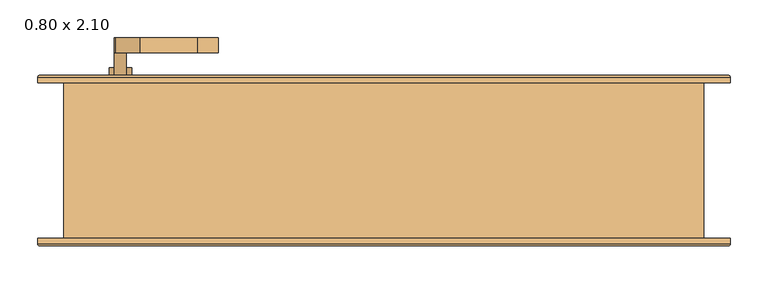
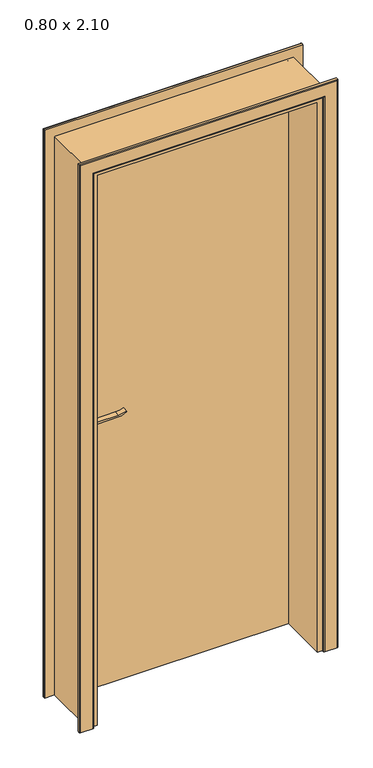
"""IFC4 building model written with IfcOpenShell, lengths in millimetres: door geometry, .CC_ND 300_PORTA SIMPLES DE ABRIR_COM EXTENSÃO : 0.80 x 2.10."""

from ifc_helpers import new_model, si_unit, point, frame, frame_2d, origin, origin_with_axes, place, context, project, spatial, polyline, circle_curve, ellipse_curve, trimmed, segment, composite_curve, outline, extrude, faceted_brep, source, transform, mapped, element, save
from ifc_brep_helpers import plane_surface, cylinder_surface, advanced_brep


def door_0_80_x_2_10_4cab1925(model_context):
    return source(origin(), model_context, "Body", "SolidModel", [
        extrude(outline(composite_curve([segment(trimmed(circle_curve(frame_2d((964.5, -350.0)), 15.0), [point((964.5, -335.0))], [point((964.5, -365.0))], False, "CARTESIAN"), True, "CONTINUOUS"), segment(trimmed(circle_curve(frame_2d((964.5, -350.0)), 15.0), [point((964.5, -365.0))], [point((964.5, -335.0))], False, "CARTESIAN"), True, "CONTINUOUS")], self_intersect=False)), frame((0.0, 110.7, 0.0), z_axis=(0.0, 1.0, 0.0), x_axis=(0.0, 0.0, 1.0)), (0.0, 0.0, 1.0), 10.0),
        extrude(outline(composite_curve([segment(trimmed(circle_curve(frame_2d((964.5, -350.0)), 15.0), [point((964.5, -335.0))], [point((964.5, -365.0))], False, "CARTESIAN"), True, "CONTINUOUS"), segment(trimmed(circle_curve(frame_2d((964.5, -350.0)), 15.0), [point((964.5, -365.0))], [point((964.5, -335.0))], False, "CARTESIAN"), True, "CONTINUOUS")], self_intersect=False)), frame((0.0, 50.7, 0.0), z_axis=(0.0, 1.0, 0.0), x_axis=(0.0, 0.0, 1.0)), (0.0, 0.0, 1.0), 10.0),
        extrude(outline(composite_curve([segment(trimmed(circle_curve(frame_2d((1024.5, -350.0)), 8.0), [point((1029.1523287, -356.5081363))], [point((1024.5, -342.0))], False, "CARTESIAN"), True, "CONTINUOUS"), segment(trimmed(circle_curve(frame_2d((1019.3738613, -324.6138099)), 18.1261387), [point((1024.5, -342.0))], [point((1037.5, -324.6138099))], True, "CARTESIAN"), True, "CONTINUOUS"), segment(polyline([(1037.5, -324.6138099), (1037.5, -248.3564091)]), True, "CONTINUOUS"), segment(trimmed(circle_curve(frame_2d((1096.7709207, -251.9396612)), 59.3791355), [point((1037.5, -248.3564091))], [point((1046.7135558, -220.0))], False, "CARTESIAN"), True, "CONTINUOUS"), segment(polyline([(1046.7135558, -220.0), (1049.5, -220.0)]), True, "CONTINUOUS"), segment(trimmed(circle_curve(frame_2d((1127.7850638, -248.4227909)), 83.2850902), [point((1049.5, -220.0))], [point((1044.5, -248.3564091))], True, "CARTESIAN"), True, "CONTINUOUS"), segment(polyline([(1044.5, -248.3564091), (1044.5, -324.6325667)]), True, "CONTINUOUS"), segment(trimmed(circle_curve(frame_2d((1007.2555521, -326.3324871)), 37.2832219), [point((1044.5, -324.6325667))], [point((1029.1523287, -356.5081363))], False, "CARTESIAN"), True, "CONTINUOUS")], self_intersect=False)), frame((0.0, 140.7, 0.0), z_axis=(0.0, 1.0, 0.0), x_axis=(0.0, 0.0, 1.0)), (0.0, 0.0, 1.0), 20.0),
        extrude(outline(composite_curve([segment(trimmed(circle_curve(frame_2d((1019.3738682, -324.6138122)), 18.1261318), [point((1024.4999903, -342.0))], [point((1037.5, -324.6138122))], True, "CARTESIAN"), True, "CONTINUOUS"), segment(polyline([(1037.5, -324.6138122), (1037.5, -248.3564091)]), True, "CONTINUOUS"), segment(trimmed(circle_curve(frame_2d((1096.7709207, -251.9396612)), 59.3791355), [point((1037.5, -248.3564091))], [point((1046.7135558, -220.0))], False, "CARTESIAN"), True, "CONTINUOUS"), segment(polyline([(1046.7135558, -220.0), (1049.5, -220.0)]), True, "CONTINUOUS"), segment(trimmed(circle_curve(frame_2d((1127.7850638, -248.4227909)), 83.2850902), [point((1049.5, -220.0))], [point((1044.5, -248.3564091))], True, "CARTESIAN"), True, "CONTINUOUS"), segment(polyline([(1044.5, -248.3564091), (1044.5, -324.6325667)]), True, "CONTINUOUS"), segment(trimmed(circle_curve(frame_2d((1007.2555521, -326.3324871)), 37.2832219), [point((1044.5, -324.6325667))], [point((1029.1523287, -356.5081363))], False, "CARTESIAN"), True, "CONTINUOUS"), segment(trimmed(circle_curve(frame_2d((1024.5, -350.0)), 8.0), [point((1029.1523287, -356.5081363))], [point((1024.4999903, -342.0))], False, "CARTESIAN"), True, "CONTINUOUS")], self_intersect=False)), frame((0.0, 10.7, 0.0), z_axis=(0.0, 1.0, 0.0), x_axis=(0.0, 0.0, 1.0)), (0.0, 0.0, 1.0), 20.0),
        extrude(outline(composite_curve([segment(trimmed(circle_curve(frame_2d((1024.5, -350.0)), 8.0), [point((1024.5, -342.0))], [point((1024.5, -358.0))], False, "CARTESIAN"), True, "CONTINUOUS"), segment(trimmed(circle_curve(frame_2d((1024.5, -350.0)), 8.0), [point((1024.5, -358.0))], [point((1024.5, -342.0))], False, "CARTESIAN"), True, "CONTINUOUS")], self_intersect=False)), frame((0.0, 110.7, 0.0), z_axis=(0.0, 1.0, 0.0), x_axis=(0.0, 0.0, 1.0)), (0.0, 0.0, 1.0), 30.0),
        extrude(outline(composite_curve([segment(trimmed(circle_curve(frame_2d((1024.5, -350.0)), 8.0), [point((1024.5, -342.0))], [point((1024.5, -358.0))], False, "CARTESIAN"), True, "CONTINUOUS"), segment(trimmed(circle_curve(frame_2d((1024.5, -350.0)), 8.0), [point((1024.5, -358.0))], [point((1024.5, -342.0))], False, "CARTESIAN"), True, "CONTINUOUS")], self_intersect=False)), frame((0.0, 30.7, 0.0), z_axis=(0.0, 1.0, 0.0), x_axis=(0.0, 0.0, 1.0)), (0.0, 0.0, 1.0), 30.0),
        extrude(outline(composite_curve([segment(trimmed(circle_curve(frame_2d((954.5, -350.0)), 25.0), [point((954.5, -375.0))], [point((954.5, -325.0))], False, "CARTESIAN"), True, "CONTINUOUS"), segment(polyline([(954.5, -325.0), (1024.5, -325.0)]), True, "CONTINUOUS"), segment(trimmed(circle_curve(frame_2d((1024.5, -350.0)), 25.0), [point((1024.5, -325.0))], [point((1024.5, -375.0))], False, "CARTESIAN"), True, "CONTINUOUS"), segment(polyline([(1024.5, -375.0), (954.5, -375.0)]), True, "CONTINUOUS")], self_intersect=False)), frame((0.0, 100.7, 0.0), z_axis=(0.0, 1.0, 0.0), x_axis=(0.0, 0.0, 1.0)), (0.0, 0.0, 1.0), 10.0),
        extrude(outline(composite_curve([segment(trimmed(circle_curve(frame_2d((954.5, -350.0)), 25.0), [point((954.5, -375.0))], [point((954.5, -325.0))], False, "CARTESIAN"), True, "CONTINUOUS"), segment(polyline([(954.5, -325.0), (1024.5, -325.0)]), True, "CONTINUOUS"), segment(trimmed(circle_curve(frame_2d((1024.5, -350.0)), 25.0), [point((1024.5, -325.0))], [point((1024.5, -375.0))], False, "CARTESIAN"), True, "CONTINUOUS"), segment(polyline([(1024.5, -375.0), (954.5, -375.0)]), True, "CONTINUOUS")], self_intersect=False)), frame((0.0, 60.7, 0.0), z_axis=(0.0, 1.0, 0.0), x_axis=(0.0, 0.0, 1.0)), (0.0, 0.0, 1.0), 10.0),
        advanced_brep(
        [(-460.0, 100.7, 0.0), (-460.0, 107.7, 0.0), (-457.0, 110.7, 0.0), (-413.0, 110.7, 0.0), (-410.0, 107.7, 0.0), (-410.0, 100.7, 0.0), (-410.0, 100.7, 2085.0), (410.0, 100.7, 2085.0), (410.0, 100.7, 0.0), (460.0, 100.7, 0.0), (460.0, 100.7, 2135.0), (-460.0, 100.7, 2135.0), (-410.0, 107.7, 2085.0), (-413.0, 110.7, 2088.0), (-457.0, 110.7, 2132.0), (457.0, 110.7, 2132.0), (457.0, 110.7, 0.0), (413.0, 110.7, 0.0), (413.0, 110.7, 2088.0), (-460.0, 107.7, 2135.0), (460.0, 107.7, 0.0), (460.0, 107.7, 2135.0), (410.0, 107.7, 0.0), (410.0, 107.7, 2085.0)],
        [
            (0, 1),
            (1, 2, circle_curve(frame((-457.0, 107.7, 0.0), z_axis=(0.0, 0.0, -1.0), x_axis=(1.0, 0.0, 0.0)), 3.0)),
            (2, 3),
            (3, 4, circle_curve(frame((-413.0, 107.7, 0.0), z_axis=(0.0, 0.0, -1.0), x_axis=(1.0, 0.0, 0.0)), 3.0)),
            (4, 5),
            (5, 0),
            (5, 6),
            (6, 7),
            (7, 8),
            (8, 9),
            (9, 10),
            (10, 11),
            (11, 0),
            (4, 12),
            (12, 6),
            (3, 13),
            (13, 12, ellipse_curve(frame((-413.0, 107.7, 2088.0), z_axis=(-0.7071067811865475, 0.0, -0.7071067811865475), x_axis=(0.7071067811865474, 0.0, -0.7071067811865476)), 4.2426407, 3.0)),
            (2, 14),
            (14, 15),
            (15, 16),
            (16, 17),
            (17, 18),
            (18, 13),
            (1, 19),
            (19, 14, ellipse_curve(frame((-457.0, 107.7, 2132.0), z_axis=(-0.7071067811865475, 0.0, -0.7071067811865475), x_axis=(0.7071067811865474, 0.0, -0.7071067811865476)), 4.2426407, 3.0)),
            (11, 19),
            (9, 20),
            (20, 21),
            (21, 10),
            (8, 22),
            (22, 17, circle_curve(frame((413.0, 107.7, 0.0), z_axis=(0.0, 0.0, -1.0), x_axis=(-1.0, 0.0, 0.0)), 3.0)),
            (16, 20, circle_curve(frame((457.0, 107.7, 0.0), z_axis=(0.0, 0.0, -1.0), x_axis=(-1.0, 0.0, 0.0)), 3.0)),
            (23, 22),
            (7, 23),
            (23, 18, ellipse_curve(frame((413.0, 107.7, 2088.0), z_axis=(0.7071067811865475, 0.0, -0.7071067811865475), x_axis=(0.7071067811865474, 0.0, 0.7071067811865476)), 4.2426407, 3.0)),
            (15, 21, ellipse_curve(frame((457.0, 107.7, 2132.0), z_axis=(0.7071067811865475, 0.0, -0.7071067811865475), x_axis=(0.7071067811865474, 0.0, 0.7071067811865476)), 4.2426407, 3.0)),
            (12, 23),
            (21, 19),
        ],
        [
            plane_surface(frame((-410.0, 100.7, 0.0), z_axis=(0.0, 0.0, -1.0), x_axis=(0.0, -1.0, 0.0))),
            plane_surface(frame((-460.0, 100.7, 0.0), z_axis=(0.0, -1.0, 0.0), x_axis=(0.0, 0.0, 1.0))),
            plane_surface(frame((-410.0, 100.7, 0.0), z_axis=(1.0, 0.0, 0.0), x_axis=(0.0, 0.0, 1.0))),
            cylinder_surface(frame((-413.0, 107.7, 0.0), z_axis=(0.0, 0.0, -1.0), x_axis=(1.0, 0.0, 0.0)), 3.0),
            plane_surface(frame((-413.0, 110.7, 0.0), z_axis=(0.0, 1.0, 0.0), x_axis=(0.0, 0.0, 1.0))),
            cylinder_surface(frame((-457.0, 107.7, 0.0), z_axis=(0.0, 0.0, -1.0), x_axis=(1.0, 0.0, 0.0)), 3.0),
            plane_surface(frame((-460.0, 107.7, 0.0), z_axis=(-1.0, 0.0, 0.0), x_axis=(0.0, 0.0, 1.0))),
            plane_surface(frame((460.0, 107.7, 2135.0), z_axis=(1.0, 0.0, 0.0), x_axis=(0.0, 0.0, -1.0))),
            plane_surface(frame((410.0, 100.7, 0.0), z_axis=(0.0, 0.0, -1.0), x_axis=(0.0, -1.0, 0.0))),
            plane_surface(frame((410.0, 100.7, 2085.0), z_axis=(-1.0, 0.0, 0.0), x_axis=(0.0, 0.0, -1.0))),
            cylinder_surface(frame((413.0, 107.7, 2085.0), z_axis=(0.0, 0.0, 1.0), x_axis=(-1.0, 0.0, 0.0)), 3.0),
            cylinder_surface(frame((457.0, 107.7, 2085.0), z_axis=(0.0, 0.0, 1.0), x_axis=(-1.0, 0.0, 0.0)), 3.0),
            plane_surface(frame((-410.0, 100.7, 2085.0), z_axis=(0.0, 0.0, -1.0), x_axis=(1.0, 0.0, 0.0))),
            plane_surface(frame((-460.0, 107.7, 2135.0), z_axis=(0.0, 0.0, 1.0), x_axis=(1.0, 0.0, 0.0))),
            cylinder_surface(frame((-410.0, 107.7, 2088.0), z_axis=(-1.0, 0.0, 0.0), x_axis=(0.0, 0.0, -1.0)), 3.0),
            cylinder_surface(frame((-410.0, 107.7, 2132.0), z_axis=(-1.0, 0.0, 0.0), x_axis=(0.0, 0.0, -1.0)), 3.0),
        ],
        [
            (0, [[1, 2, 3, 4, 5, 6]]),
            (1, [[7, 8, 9, 10, 11, 12, 13, -6]]),
            (2, [[14, 15, -7, -5]]),
            (3, [[16, 17, -14, -4]]),
            (4, [[18, 19, 20, 21, 22, 23, -16, -3]]),
            (5, [[24, 25, -18, -2]]),
            (6, [[-13, 26, -24, -1]]),
            (7, [[-11, 27, 28, 29]]),
            (8, [[-10, 30, 31, -21, 32, -27]]),
            (9, [[33, -30, -9, 34]]),
            (10, [[-22, -31, -33, 35]]),
            (11, [[-28, -32, -20, 36]]),
            (12, [[37, -34, -8, -15]]),
            (13, [[-12, -29, 38, -26]]),
            (14, [[-23, -35, -37, -17]]),
            (15, [[-38, -36, -19, -25]]),
        ],
    ),
        advanced_brep(
        [(460.0, -106.0, 0.0), (460.0, -113.0342217, 0.0), (457.0342217, -116.0, 0.0), (412.9842717, -116.0, 0.0), (410.0, -113.0157283, 0.0), (410.0, -106.0, 0.0), (410.0, -106.0, 2085.0), (-410.0, -106.0, 2085.0), (-410.0, -106.0, 0.0), (-460.0, -106.0, 0.0), (-460.0, -106.0, 2135.0), (460.0, -106.0, 2135.0), (410.0, -113.0157283, 2085.0), (412.9842717, -116.0, 2087.9842717), (457.0342217, -116.0, 2132.0342217), (-457.0342217, -116.0, 2132.0342217), (-457.0342217, -116.0, 0.0), (-412.9842717, -116.0, 0.0), (-412.9842717, -116.0, 2087.9842717), (460.0, -113.0342217, 2135.0), (-460.0, -113.0342217, 0.0), (-460.0, -113.0342217, 2135.0), (-410.0, -113.0157283, 0.0), (-410.0, -113.0157283, 2085.0)],
        [
            (0, 1),
            (1, 2, circle_curve(frame((457.0342217, -113.0342217, 0.0), z_axis=(0.0, 0.0, -1.0), x_axis=(1.0, 0.0, 0.0)), 2.9657783)),
            (2, 3),
            (3, 4, circle_curve(frame((412.9842717, -113.0157283, 0.0), z_axis=(0.0, 0.0, -1.0), x_axis=(1.0, 0.0, 0.0)), 2.9842717)),
            (4, 5),
            (5, 0),
            (5, 6),
            (6, 7),
            (7, 8),
            (8, 9),
            (9, 10),
            (10, 11),
            (11, 0),
            (4, 12),
            (12, 6),
            (3, 13),
            (13, 12, ellipse_curve(frame((412.9842717, -113.0157283, 2087.9842717), z_axis=(0.7071067811865475, 0.0, -0.7071067811865475), x_axis=(-0.7071067811865474, 0.0, -0.7071067811865476)), 4.2203975, 2.9842717)),
            (2, 14),
            (14, 15),
            (15, 16),
            (16, 17),
            (17, 18),
            (18, 13),
            (1, 19),
            (19, 14, ellipse_curve(frame((457.0342217, -113.0342217, 2132.0342217), z_axis=(0.7071067811865475, 0.0, -0.7071067811865475), x_axis=(-0.7071067811865474, 0.0, -0.7071067811865476)), 4.1942438, 2.9657783)),
            (11, 19),
            (9, 20),
            (20, 21),
            (21, 10),
            (8, 22),
            (22, 17, circle_curve(frame((-412.9842717, -113.0157283, 0.0), z_axis=(0.0, 0.0, -1.0), x_axis=(-1.0, 0.0, 0.0)), 2.9842717)),
            (16, 20, circle_curve(frame((-457.0342217, -113.0342217, 0.0), z_axis=(0.0, 0.0, -1.0), x_axis=(-1.0, 0.0, 0.0)), 2.9657783)),
            (23, 22),
            (7, 23),
            (23, 18, ellipse_curve(frame((-412.9842717, -113.0157283, 2087.9842717), z_axis=(-0.7071067811865475, 0.0, -0.7071067811865475), x_axis=(-0.7071067811865474, 0.0, 0.7071067811865476)), 4.2203975, 2.9842717)),
            (15, 21, ellipse_curve(frame((-457.0342217, -113.0342217, 2132.0342217), z_axis=(-0.7071067811865475, 0.0, -0.7071067811865475), x_axis=(-0.7071067811865474, 0.0, 0.7071067811865476)), 4.1942438, 2.9657783)),
            (12, 23),
            (21, 19),
        ],
        [
            plane_surface(frame((410.0, -106.0, 0.0), z_axis=(0.0, 0.0, -1.0), x_axis=(0.0, -1.0, 0.0))),
            plane_surface(frame((460.0, -106.0, 0.0), z_axis=(0.0, 1.0, 0.0), x_axis=(0.0, 0.0, 1.0))),
            plane_surface(frame((410.0, -106.0, 0.0), z_axis=(-1.0, 0.0, 0.0), x_axis=(0.0, 0.0, 1.0))),
            cylinder_surface(frame((412.9842717, -113.0157283, 0.0), z_axis=(0.0, 0.0, -1.0), x_axis=(1.0, 0.0, 0.0)), 2.9842717),
            plane_surface(frame((412.9842717, -116.0, 0.0), z_axis=(0.0, -1.0, 0.0), x_axis=(0.0, 0.0, 1.0))),
            cylinder_surface(frame((457.0342217, -113.0342217, 0.0), z_axis=(0.0, 0.0, -1.0), x_axis=(1.0, 0.0, 0.0)), 2.9657783),
            plane_surface(frame((460.0, -113.0342217, 0.0), z_axis=(1.0, 0.0, 0.0), x_axis=(0.0, 0.0, 1.0))),
            plane_surface(frame((-460.0, -113.0342217, 2135.0), z_axis=(-1.0, 0.0, 0.0), x_axis=(0.0, 0.0, -1.0))),
            plane_surface(frame((-410.0, -106.0, 0.0), z_axis=(0.0, 0.0, -1.0), x_axis=(0.0, -1.0, 0.0))),
            plane_surface(frame((-410.0, -106.0, 2085.0), z_axis=(1.0, 0.0, 0.0), x_axis=(0.0, 0.0, -1.0))),
            cylinder_surface(frame((-412.9842717, -113.0157283, 2085.0), z_axis=(0.0, 0.0, 1.0), x_axis=(-1.0, 0.0, 0.0)), 2.9842717),
            cylinder_surface(frame((-457.0342217, -113.0342217, 2085.0), z_axis=(0.0, 0.0, 1.0), x_axis=(-1.0, 0.0, 0.0)), 2.9657783),
            plane_surface(frame((410.0, -106.0, 2085.0), z_axis=(0.0, 0.0, -1.0), x_axis=(-1.0, 0.0, 0.0))),
            plane_surface(frame((460.0, -113.0342217, 2135.0), z_axis=(0.0, 0.0, 1.0), x_axis=(-1.0, 0.0, 0.0))),
            cylinder_surface(frame((410.0, -113.0157283, 2087.9842717), z_axis=(1.0, 0.0, 0.0), x_axis=(0.0, 0.0, 1.0)), 2.9842717),
            cylinder_surface(frame((410.0, -113.0342217, 2132.0342217), z_axis=(1.0, 0.0, 0.0), x_axis=(0.0, 0.0, 1.0)), 2.9657783),
        ],
        [
            (0, [[1, 2, 3, 4, 5, 6]]),
            (1, [[7, 8, 9, 10, 11, 12, 13, -6]]),
            (2, [[14, 15, -7, -5]]),
            (3, [[16, 17, -14, -4]]),
            (4, [[18, 19, 20, 21, 22, 23, -16, -3]]),
            (5, [[24, 25, -18, -2]]),
            (6, [[-13, 26, -24, -1]]),
            (7, [[-11, 27, 28, 29]]),
            (8, [[-10, 30, 31, -21, 32, -27]]),
            (9, [[33, -30, -9, 34]]),
            (10, [[-22, -31, -33, 35]]),
            (11, [[-28, -32, -20, 36]]),
            (12, [[37, -34, -8, -15]]),
            (13, [[-12, -29, 38, -26]]),
            (14, [[-23, -35, -37, -17]]),
            (15, [[-38, -36, -19, -25]]),
        ],
    ),
        faceted_brep([(392.0, -106.0, 0.0), (392.0, 70.7, 0.0), (400.0, 70.7, 0.0), (400.0, 100.7, 0.0), (425.0, 100.7, 0.0), (425.0, -106.0, 0.0), (425.0, -106.0, 2100.0), (-425.0, -106.0, 2100.0), (-425.0, -106.0, 0.0), (-392.0, -106.0, 0.0), (-392.0, -106.0, 2067.0), (392.0, -106.0, 2067.0), (425.0, 100.7, 2100.0), (400.0, 100.7, 2075.0), (-400.0, 100.7, 2075.0), (-400.0, 100.7, 0.0), (-425.0, 100.7, 0.0), (-425.0, 100.7, 2100.0), (400.0, 70.7, 2075.0), (392.0, 70.7, 2067.0), (-392.0, 70.7, 2067.0), (-392.0, 70.7, 0.0), (-400.0, 70.7, 0.0), (-400.0, 70.7, 2075.0)], [[[0, 1, 2, 3, 4, 5]], [[5, 6, 7, 8, 9, 10, 11, 0]], [[4, 12, 6, 5]], [[3, 13, 14, 15, 16, 17, 12, 4]], [[2, 18, 13, 3]], [[1, 19, 20, 21, 22, 23, 18, 2]], [[0, 11, 19, 1]], [[10, 9, 21, 20]], [[9, 8, 16, 15, 22, 21]], [[17, 16, 8, 7]], [[23, 22, 15, 14]], [[12, 17, 7, 6]], [[18, 23, 14, 13]], [[11, 10, 20, 19]]]),
        extrude(outline(polyline([(-400.0, 70.7), (-400.0, 100.7), (400.0, 100.7), (400.0, 70.7), (-400.0, 70.7)])), origin_with_axes(), (0.0, 0.0, 1.0), 2075.0),
    ])


if __name__ == "__main__":
    model = new_model("IFC4")
    model_context = context("Model", 3, world=origin())
    ifc_project = project(units=[si_unit("LENGTHUNIT", "METRE", prefix="MILLI")], contexts=[model_context])
    site = spatial("IfcSite", under=ifc_project)
    building = spatial("IfcBuilding", under=site)
    placement = place(None, origin())
    door_0_80_x_2_10_shape = door_0_80_x_2_10_4cab1925(model_context)
    element("IfcDoor", 1, ObjectType=".CC_ND 300_PORTA SIMPLES DE ABRIR_COM EXTENSÃO : 0.80 x 2.10", at=placement, inside=building, context=model_context, shape_type="MappedRepresentation", body=[
        mapped(door_0_80_x_2_10_shape, transform((0.0, 0.0, 0.0), x_axis=(1.0, 0.0, 0.0), y_axis=(0.0, 1.0, 0.0), z_axis=(0.0, 0.0, 1.0))),
    ])
    save(model, "model.ifc")

# Revit data of these elements
# Type ".CC_ND 300_PORTA SIMPLES DE ABRIR_COM EXTENSÃO : 0.80 x 2.10"
#   Type Mark = "153"
#   Rough Width = 0.85 m
#   Espessura moldura externa = 0.01 m
#   Espessura moldura interna = 0.01 m
#   Largura moldura = 0.05 m
#   Extensão acabamento exterior [instance default] = 0.00 m
#   Extensão acabamento interior [instance default] = 0.00 m
#   Espessura batente = 0.025 m
#   Thickness = 0.03 m
#   Altura batente = 2.085 m
#   Aux Arco [instance default] = 0.80 m
#   Rough Height = 2.125 m
#   Height = 2.10 m
#   Width = 0.80 m
#   Moldura interna [instance default] = yes
#   Moldura externa [instance default] = yes
#   Porta = .MADEIRA COM PINTURA ESMALTE BRANCO ACETINADO
#   Moldura = .MADEIRA COM PINTURA ESMALTE BRANCO ACETINADO
#   Maçaneta = .ALUMÍNIO
#   Batente = .MADEIRA COM PINTURA ESMALTE BRANCO ACETINADO
#   Function = (empty or 0)
#   Wall Closure = (empty or 0)
# Element 1 (IfcDoor, ".CC_ND 300_PORTA SIMPLES DE ABRIR_COM EXTENSÃO : 0.80 x 2.10")
#   Extensão acabamento exterior = 0.031 m
#   Extensão acabamento interior = 0.0257 m
#   Aux Arco = 0.8257 m
#   Materials on its faces: ".MADEIRA COM PINTURA ESMALTE BRANCO ACETINADO", ".ALUMÍNIO"
# Materials
#   ".MADEIRA COM PINTURA ESMALTE BRANCO ACETINADO": class ".CC_MADEIRAS", colour RGB 240 240 240, transparency 0, Description = "Madeira com pintura esmalte branco acetinado.", Cost = 0
#   ".ALUMÍNIO": class "CC_METAIS", colour RGB 244 244 244, transparency 0, Description = "Material alumínio", Cost = 0
